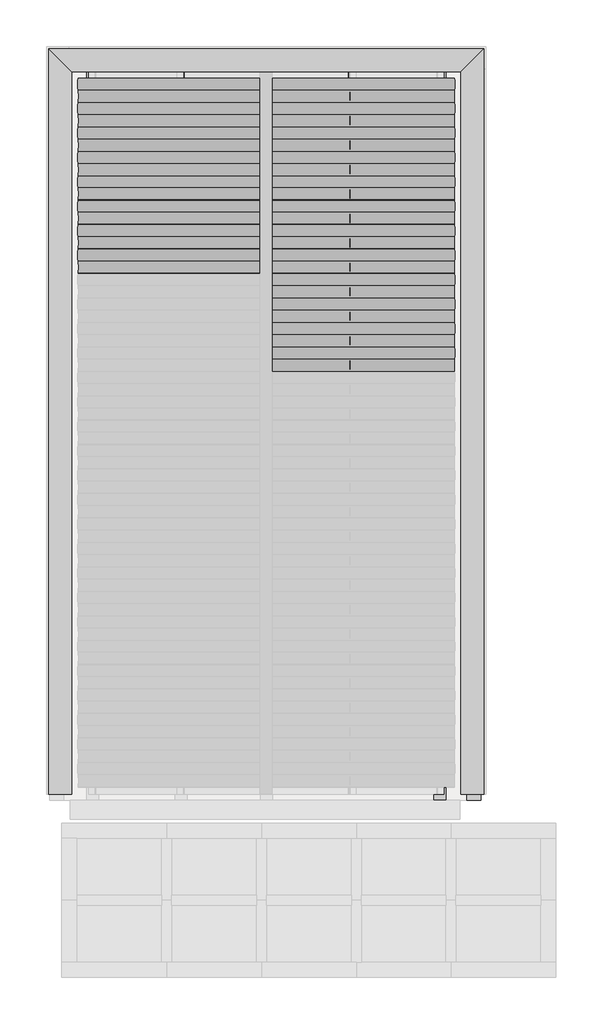
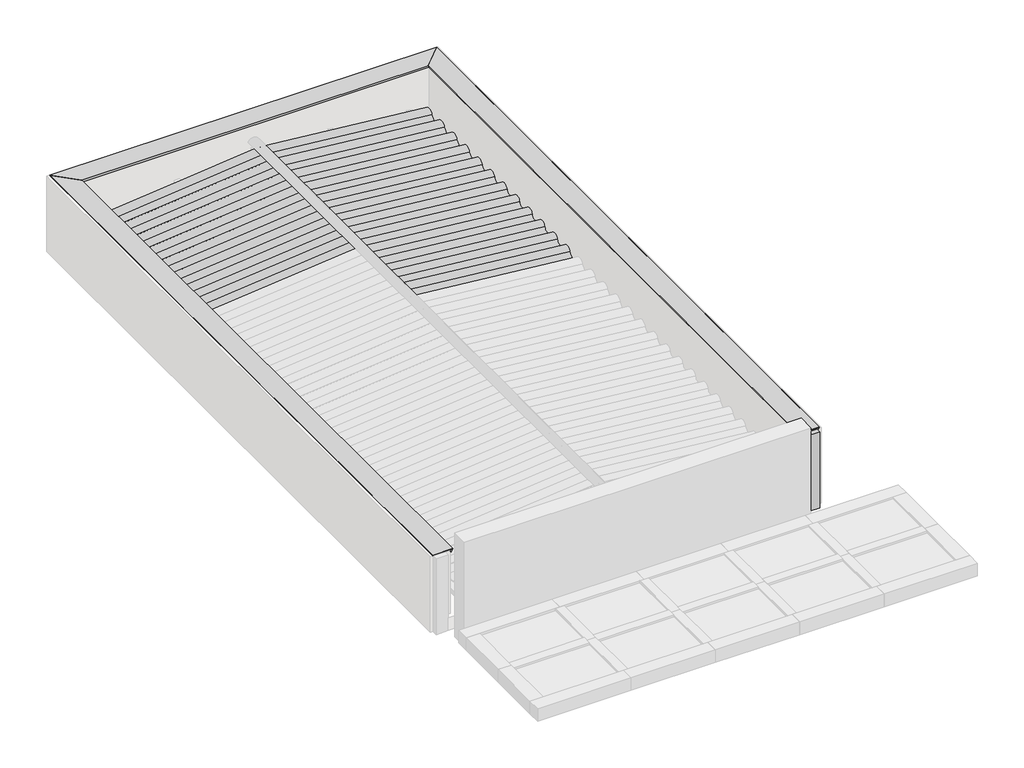
# One storey, part 3 of 3: 35 beams, 12 columns, 1 proxy.
# Revit data of these elements (continued)
# Element 14 (IfcBeam, "TQS - Viga retangular : 14.0 x 90.0") (continued)
#   Resultado de Ensaios fck (MPa) = 0
#   Unique TQS ID = -1268
#   Principal = yes
#   Structural Material = none
#   Phase Created = CC_PE
# Element 15 (IfcBeam, "TQS - Viga retangular : 14.0 x 90.0")
#   Uso = "ESTRUTURA"
#   Titulo = "V104"
#   Chave = "-1270"
#   Tipo Elemento = "Viga"
#   SHA1 = "0A21AF0D9A5F34D6093C65F9A93BBB9D744C094D"
#   Revisão = ""
#   Tipo de carga = ""
#   Divisor de flexao = ""
#   Secao = ""
#   Configuracao = ""
#   Angulo (graus) = ""
#   Detalhamento = ""
#   Casos de vento manual = ""
#   Tipo = ""
#   Alcas = ""
#   Furos = ""
#   Pino = ""
#   Distribuicao = ""
#   Solidarizado = ""
#   Solidarizar na montagem = ""
#   Unir com o próximo = ""
#   Grupo pre moldado = ""
#   Verificado = ""
#   Concreto C = ""
#   Taxa de armadura (kgf/m³) = 0
#   Carga (tf/m²) = 0
#   Carga (tf/m) = 0
#   Carga (tf) = 0
#   Altura = 0.90 m
#   Rebaixo = -0.75 m
#   Largura = 0.14 m
#   Distancia a face = 0.00 m
#   Distancia ao eixo = 0.00 m
#   Altura gerber esquerda = 0.00 m
#   Largura gerber esquerda = 0.00 m
#   Altura gerber direita = 0.00 m
#   Largura gerber direita = 0.00 m
#   Resultado de Ensaios fck (MPa) = 0
#   Unique TQS ID = -1270
#   Principal = yes
#   Structural Material = none
#   Phase Created = CC_PE
# Elements 16, 17, 18, 19, 20, 21, 22, 23, 24, 25, 26, 27, 28, 29, 30, 31, 32, 33, 34, 35 (IfcBeam, "Telha Ondulada : Fibrocimento")
#   Uso = "TELHADOS TELHAS"
#   Phase Created = CC_AP
#   Materials on its faces: ".TELHA DE FIBROCIMENTO"
# Element 36 (IfcBuildingElementProxy, ".CC_RUFO_PINGADEIRA_22 cm")
#   Uso = "RUFOS COB. GARAGEM"
#   Phase Created = CC_PE
#   Materials on its faces: ".ALUMÍNIO COM PINTURA LÁTEX BRANCA"
# Elements 37, 38, 39, 40, 41, 42, 43, 44, 45, 46, 47, 48 (IfcColumn, "Madeira de lei-Coluna : Pontalete 6X16cm")
#   Comments = ""
#   Uso = "TELHADOS ESTRUTURAS"
#   Compr Cmcl = 2.00 m
#   Structural Material = .MADEIRAMENTO
#   Phase Created = CC_AP
#   Materials on its faces: ".MADEIRAMENTO"
# Materials
#   ".TELHA DE FIBROCIMENTO": class "CC_TELHADO", colour RGB 77 77 76, transparency 0, Description = "TELHA ONDULADA FIBROCIMENTO", Cost = 0
#   ".MADEIRAMENTO": class ".CC_MADEIRAS", colour RGB 212 179 113, transparency 0, Cost = 0
#   ".ALUMÍNIO COM PINTURA LÁTEX BRANCA": class "Generic", colour RGB 250 250 250, transparency 0, Cost = 0
